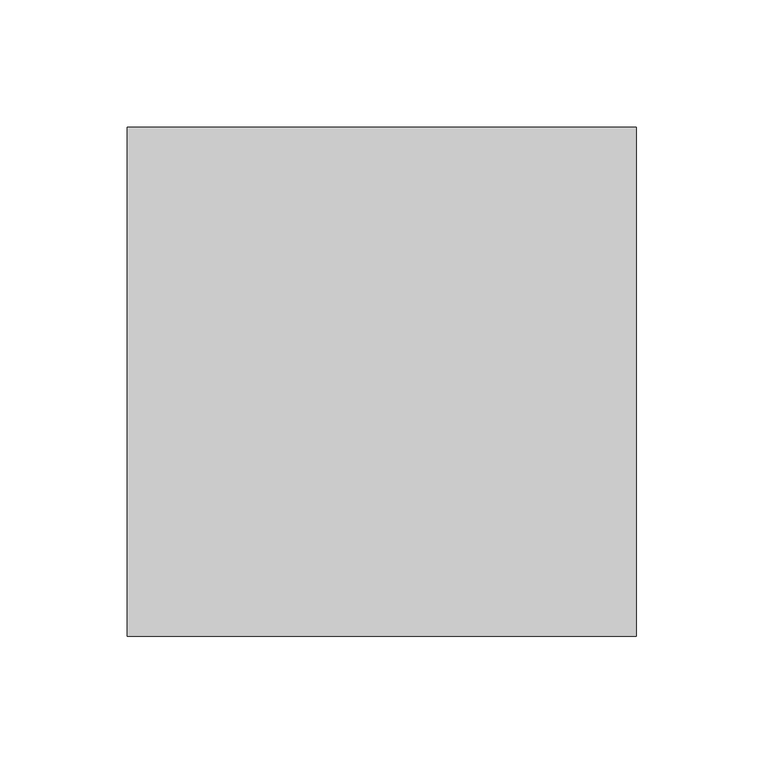
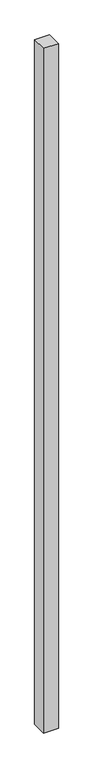
"""IFC4 building model written with IfcOpenShell, lengths in millimetres: column geometry, 0_3d."""

import ifcopenshell
import ifcopenshell.guid

model = None  # the IFC model being written
_history = None  # IfcOwnerHistory: only IFC2X3 demands one
_inside = {}  # id of a spatial element -> (the spatial element, [elements in it])
_under = {}  # id of a project, library or spatial element -> (it, [spatial elements below it])
_declared = {}  # id of a project -> (the project, [libraries it declares])
_typed = {}  # id of a type object -> (the type object, [elements of that type])
_made_of = {}  # id of a material, layer set ... -> (it, [elements and type objects made of it])


def new_model(schema):
    """Start an empty IFC model of exactly this schema.

    Asked for "IFC4X3", IfcOpenShell would pick the latest addendum, in which some entities
    have other attributes; the version numbers below select the first issue.
    IFC2X3 requires an IfcOwnerHistory on every rooted entity: one is made here for all.
    """
    global model, _history
    if schema == "IFC4X3":
        model = ifcopenshell.file(schema_version=(4, 3, 0, 0))
    else:
        model = ifcopenshell.file(schema=schema)
    _inside.clear()
    _under.clear()
    _declared.clear()
    _typed.clear()
    _made_of.clear()
    _history = None
    if model.schema == "IFC2X3":
        org = make("IfcOrganization", Name="unknown")
        user = make(
            "IfcPersonAndOrganization",
            ThePerson=make("IfcPerson", FamilyName="unknown"),
            TheOrganization=org,
        )
        app = make(
            "IfcApplication",
            ApplicationDeveloper=org,
            Version="unknown",
            ApplicationFullName="unknown",
            ApplicationIdentifier="unknown",
        )
        _history = make(
            "IfcOwnerHistory",
            OwningUser=user,
            OwningApplication=app,
            ChangeAction="ADDED",
            CreationDate=0,
        )
    return model


def make(cls, **values):
    """One entity of the class cls with the attributes given. An attribute that is None is left unset."""
    return model.create_entity(
        cls, **{name: value for name, value in values.items() if value is not None}
    )


def rooted(cls, **values):
    """An entity with a GlobalId (a new one), such as an element, a storey or a relation."""
    return make(cls, GlobalId=ifcopenshell.guid.new(), OwnerHistory=_history, **values)


def si_unit(unit_type, name, prefix=None):
    """IfcSIUnit, for example si_unit("LENGTHUNIT", "METRE", prefix="MILLI")."""
    return make("IfcSIUnit", UnitType=unit_type, Prefix=prefix, Name=name)


def assignment(units):
    """IfcUnitAssignment: the units of a project."""
    return None if units is None else make("IfcUnitAssignment", Units=units)


def point(xyz):
    """IfcCartesianPoint."""
    return None if xyz is None else make("IfcCartesianPoint", Coordinates=xyz)


def direction(xyz):
    """IfcDirection."""
    return None if xyz is None else make("IfcDirection", DirectionRatios=xyz)


def frame(location, z_axis=None, x_axis=None):
    """IfcAxis2Placement3D, a coordinate frame: its origin and axes. An axis left out is left unset."""
    return make(
        "IfcAxis2Placement3D",
        Location=point(location),
        Axis=direction(z_axis),
        RefDirection=direction(x_axis),
    )


def origin():
    """The frame at (0, 0, 0) with its axes left unset."""
    return frame((0.0, 0.0, 0.0))


def origin_with_axes():
    """The frame at (0, 0, 0) with the z axis (0, 0, 1) and the x axis (1, 0, 0) written out."""
    return frame((0.0, 0.0, 0.0), z_axis=(0.0, 0.0, 1.0), x_axis=(1.0, 0.0, 0.0))


def place(relative_to, where):
    """IfcLocalPlacement: puts the frame where relative to a parent placement (None: the world)."""
    return make(
        "IfcLocalPlacement", PlacementRelTo=relative_to, RelativePlacement=where
    )


def context(
    kind, dimensions, precision=None, world=None, true_north=None, identifier=None
):
    """IfcGeometricRepresentationContext, for example the 3D "Model" context."""
    return make(
        "IfcGeometricRepresentationContext",
        ContextIdentifier=identifier,
        ContextType=kind,
        CoordinateSpaceDimension=dimensions,
        Precision=precision,
        WorldCoordinateSystem=world,
        TrueNorth=true_north,
    )


def project(units=None, contexts=None):
    """IfcProject with its units and contexts."""
    return rooted(
        "IfcProject",
        Name="project",
        RepresentationContexts=contexts,
        UnitsInContext=assignment(units),
    )


def spatial(cls, under=None, at=None, **own):
    """A site, building, storey or space (cls), placed at a placement, below another one or the project."""
    s = rooted(cls, ObjectPlacement=at, **own)
    if under is not None:
        _under.setdefault(under.id(), (under, []))[1].append(s)
    return s


def polyline(points):
    """IfcPolyline through the points."""
    return make("IfcPolyline", Points=[point(p) for p in points])


def outline(outer, holes=None, kind="AREA"):
    """IfcArbitraryClosedProfileDef: a profile drawn as a closed curve; with holes, ...WithVoids."""
    if holes is None:
        return make("IfcArbitraryClosedProfileDef", ProfileType=kind, OuterCurve=outer)
    return make(
        "IfcArbitraryProfileDefWithVoids",
        ProfileType=kind,
        OuterCurve=outer,
        InnerCurves=holes,
    )


def extrude(swept, where, along, depth):
    """IfcExtrudedAreaSolid: the profile swept, set in the frame where, extruded along a direction by depth."""
    return make(
        "IfcExtrudedAreaSolid",
        SweptArea=swept,
        Position=where,
        ExtrudedDirection=direction(along),
        Depth=depth,
    )


def shape(context_of_items, identifier, shape_type, items):
    """IfcShapeRepresentation: the items that make up one representation, for example the "Body"."""
    return make(
        "IfcShapeRepresentation",
        ContextOfItems=context_of_items,
        RepresentationIdentifier=identifier,
        RepresentationType=shape_type,
        Items=items,
    )


def source(mapping_origin, context_of_items, identifier, shape_type, items):
    """IfcRepresentationMap: a shape defined once, which mapped items show again and again."""
    return make(
        "IfcRepresentationMap",
        MappingOrigin=mapping_origin,
        MappedRepresentation=shape(context_of_items, identifier, shape_type, items),
    )


def transform(
    local_origin,
    x_axis=None,
    y_axis=None,
    z_axis=None,
    scale=None,
    scale2=None,
    scale3=None,
    uniform=True,
):
    """IfcCartesianTransformationOperator3D, or its non-uniform kind. x_axis, y_axis, z_axis: its Axis1, 2, 3."""
    if uniform:
        return make(
            "IfcCartesianTransformationOperator3D",
            Axis1=direction(x_axis),
            Axis2=direction(y_axis),
            LocalOrigin=point(local_origin),
            Scale=scale,
            Axis3=direction(z_axis),
        )
    return make(
        "IfcCartesianTransformationOperator3DnonUniform",
        Axis1=direction(x_axis),
        Axis2=direction(y_axis),
        LocalOrigin=point(local_origin),
        Scale=scale,
        Axis3=direction(z_axis),
        Scale2=scale2,
        Scale3=scale3,
    )


def mapped(mapping_source, mapping_target):
    """IfcMappedItem: shows the shape of a source again, moved by a transform."""
    return make(
        "IfcMappedItem", MappingSource=mapping_source, MappingTarget=mapping_target
    )


def made_of(thing, what):
    """Note that an element or type object is made of a material, layer set ...; save() writes the relation."""
    if what is not None:
        _made_of.setdefault(what.id(), (what, []))[1].append(thing)
    return thing


def element(
    cls,
    number,
    at=None,
    inside=None,
    cuts=None,
    type_object=None,
    material=None,
    context=None,
    identifier="Body",
    shape_type=None,
    held_by="IfcProductDefinitionShape",
    body=None,
    shapes=None,
    **own,
):
    """One element of the class cls, such as IfcWall. Its Tag is "e" and its number.

    at: its placement. inside: the storey or other place that contains it. cuts: it is an
    opening in that element (IfcRelVoidsElement). A single representation is given by context,
    identifier, shape_type and body (its items); several are given by shapes. held_by: the class
    of the entity that holds the representations. save() writes the other relations.
    """
    e = rooted(cls, Tag="e%d" % number, ObjectPlacement=at, **own)
    if body is not None:
        shapes = [shape(context, identifier, shape_type, body)]
    if shapes is not None:
        e.Representation = make(held_by, Representations=shapes)
    if inside is not None:
        _inside.setdefault(inside.id(), (inside, []))[1].append(e)
    if cuts is not None:
        rooted(
            "IfcRelVoidsElement", RelatingBuildingElement=cuts, RelatedOpeningElement=e
        )
    if type_object is not None:
        _typed.setdefault(type_object.id(), (type_object, []))[1].append(e)
    return made_of(e, material)


def aggregate(whole, parts):
    """IfcRelAggregates: a whole, such as a stair, and the parts it consists of."""
    return rooted("IfcRelAggregates", RelatingObject=whole, RelatedObjects=parts)


def save(model, path):
    """Write the relations noted so far, then the file.

    IfcRelAggregates (storeys below a building ...), IfcRelContainedInSpatialStructure (elements
    in a storey), IfcRelDefinesByType, IfcRelAssociatesMaterial and IfcRelDeclares: one each for
    every whole, place, type object, material and project.
    """
    for whole, parts in _under.values():
        aggregate(whole, parts)
    for where, things in _inside.values():
        rooted(
            "IfcRelContainedInSpatialStructure",
            RelatedElements=things,
            RelatingStructure=where,
        )
    for kind, things in _typed.values():
        rooted("IfcRelDefinesByType", RelatedObjects=things, RelatingType=kind)
    for what, things in _made_of.values():
        rooted("IfcRelAssociatesMaterial", RelatedObjects=things, RelatingMaterial=what)
    for by, libraries in _declared.values():
        rooted("IfcRelDeclares", RelatingContext=by, RelatedDefinitions=libraries)
    model.write(path)


def column_bf906614(model_context):
    return source(origin(), model_context, "Body", "SweptSolid", [
        extrude(outline(polyline([(0.0, 200.0), (200.0, 200.0), (200.0, 0.0), (0.0, 0.0), (0.0, 200.0)])), origin_with_axes(), (0.0, 0.0, 1.0), 9650.0),
    ])


if __name__ == "__main__":
    model = new_model("IFC4")
    model_context = context("Model", 3, world=origin())
    ifc_project = project(units=[si_unit("LENGTHUNIT", "METRE", prefix="MILLI")], contexts=[model_context])
    site = spatial("IfcSite", under=ifc_project)
    building = spatial("IfcBuilding", under=site)
    placement = place(None, origin())
    column_shape = column_bf906614(model_context)
    element("IfcColumn", 1, ObjectType="0_3d", at=placement, inside=building, context=model_context, shape_type="MappedRepresentation", body=[
        mapped(column_shape, transform((0.0, 0.0, 0.0), x_axis=(1.0, 0.0, 0.0), y_axis=(0.0, 1.0, 0.0), z_axis=(0.0, 0.0, 1.0))),
    ])
    save(model, "model.ifc")

# Revit data of these elements
# Element 1 (IfcColumn, "0_3d")
#   Materials on its faces: "material wardrobe b 1"
# Materials
#   "material wardrobe b 1": class "Unassigned", colour RGB 128 128 128, transparency 0
